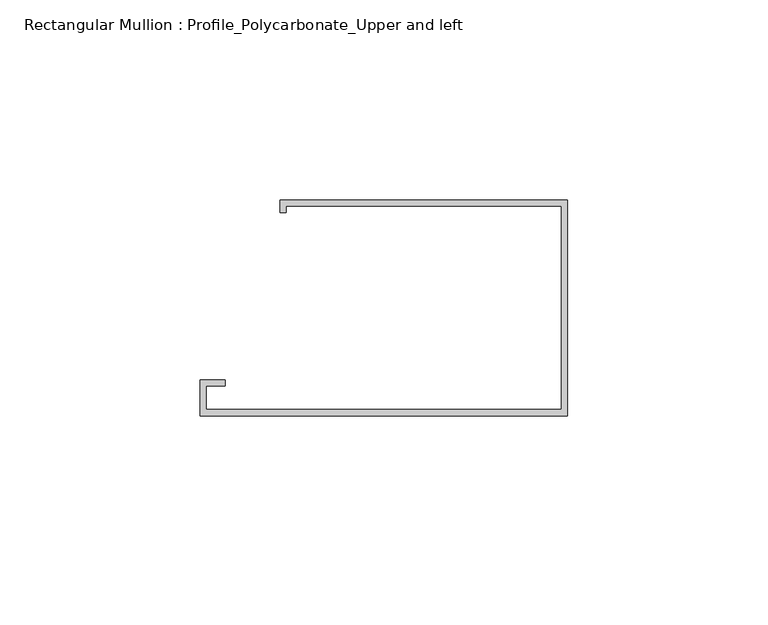
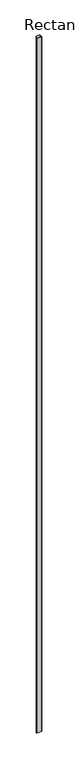
"""IFC4 building model written with IfcOpenShell, lengths in millimetres: member geometry, Rectangular Mullion : Profile_Polycarbonate_Upper and left."""

from ifc_helpers import new_model, si_unit, frame, origin, place, context, project, spatial, polyline, outline, extrude, source, transform, mapped, element, save


def rectangular_mullion_profile_polycarbonate_upper_and_left_c7642290(model_context):
    return source(origin(), model_context, "Body", "SweptSolid", [
        extrude(outline(polyline([(0.0, -28.984575), (-91.9988, -28.984575), (-91.9988, -19.992975), (-85.6488, -19.992975), (-85.6488, -21.580475), (-90.4113, -21.580475), (-90.4113, -27.397075), (-1.5875, -27.397075), (-1.5875, 23.428325), (-70.3961, 23.428325), (-70.3961, 21.840825), (-71.9836, 21.840825), (-71.9836, 25.015825), (0.0, 25.015825), (0.0, -28.984575)])), frame((0.0, 0.0, -13290.7024), z_axis=(0.0, 0.0, 1.0), x_axis=(1.0, 0.0, 0.0)), (0.0, 0.0, 1.0), 13290.7024),
    ])


if __name__ == "__main__":
    model = new_model("IFC4")
    model_context = context("Model", 3, world=origin())
    ifc_project = project(units=[si_unit("LENGTHUNIT", "METRE", prefix="MILLI")], contexts=[model_context])
    site = spatial("IfcSite", under=ifc_project)
    building = spatial("IfcBuilding", under=site)
    placement = place(None, origin())
    rectangular_mullion_profile_polycarbonate_upper_and_left_shape = rectangular_mullion_profile_polycarbonate_upper_and_left_c7642290(model_context)
    element("IfcMember", 1, ObjectType="Rectangular Mullion : Profile_Polycarbonate_Upper and left", at=placement, inside=building, context=model_context, shape_type="MappedRepresentation", body=[
        mapped(rectangular_mullion_profile_polycarbonate_upper_and_left_shape, transform((0.0, 0.0, 0.0), x_axis=(1.0, 0.0, 0.0), y_axis=(0.0, 1.0, 0.0), z_axis=(0.0, 0.0, 1.0))),
    ])
    save(model, "model.ifc")

# Revit data of these elements
# Type "Rectangular Mullion : Profile_Polycarbonate_Upper and left"
#   built-in parameter 1007322 = 0.177167 (stored number, unit not read)
#   built-in parameter 1007321 = 0.00520833 (stored number, unit not read)
#   built-in parameter 1007320 = 0 (stored number, unit not read)
